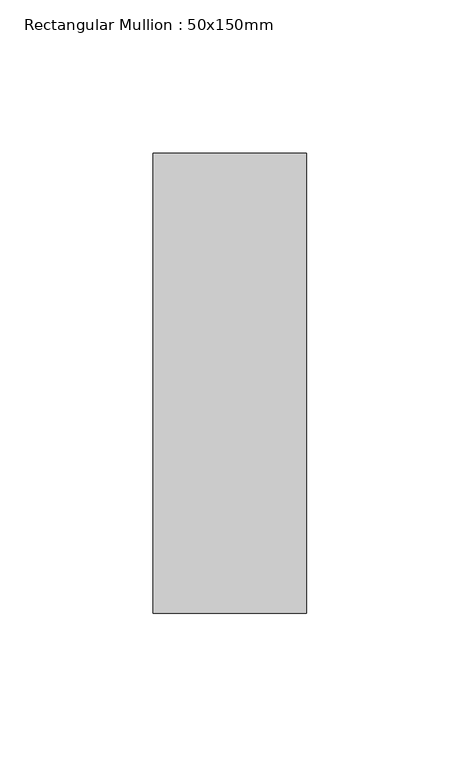
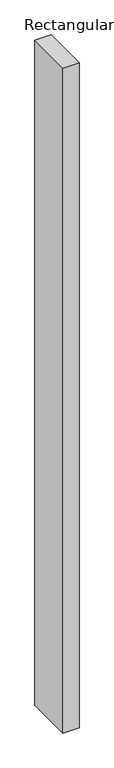
"""IFC4 building model written with IfcOpenShell, lengths in millimetres: member geometry, Rectangular Mullion : 50x150mm."""

from ifc_helpers import new_model, si_unit, frame, origin, place, context, project, spatial, polyline, outline, extrude, source, transform, mapped, element, save


def rectangular_mullion_50x150mm_0a54999a(model_context):
    return source(origin(), model_context, "Body", "SweptSolid", [
        extrude(outline(polyline([(0.0, 75.0), (0.0, -75.0), (-50.0, -75.0), (-50.0, 75.0), (0.0, 75.0)])), frame((0.0, 0.0, -2175.0), z_axis=(0.0, 0.0, 1.0), x_axis=(1.0, 0.0, 0.0)), (0.0, 0.0, 1.0), 2175.0),
    ])


if __name__ == "__main__":
    model = new_model("IFC4")
    model_context = context("Model", 3, world=origin())
    ifc_project = project(units=[si_unit("LENGTHUNIT", "METRE", prefix="MILLI")], contexts=[model_context])
    site = spatial("IfcSite", under=ifc_project)
    building = spatial("IfcBuilding", under=site)
    placement = place(None, origin())
    rectangular_mullion_50x150mm_shape = rectangular_mullion_50x150mm_0a54999a(model_context)
    element("IfcMember", 1, ObjectType="Rectangular Mullion : 50x150mm", at=placement, inside=building, context=model_context, shape_type="MappedRepresentation", body=[
        mapped(rectangular_mullion_50x150mm_shape, transform((0.0, 0.0, 0.0), x_axis=(1.0, 0.0, 0.0), y_axis=(0.0, 1.0, 0.0), z_axis=(0.0, 0.0, 1.0))),
    ])
    save(model, "model.ifc")

# Revit data of these elements
# Type "Rectangular Mullion : 50x150mm"
#   Keynote = "H11"
#   built-in parameter 1007304 = 0.492126 (stored number, unit not read)
#   built-in parameter 1007301 = 0.082021 (stored number, unit not read)
#   built-in parameter 1007300 = 0.082021 (stored number, unit not read)
# Element 1 (IfcMember, "Rectangular Mullion : 50x150mm")
#   Materials on its faces: "Aluminium"
# Materials
#   "Aluminium": class "Metal", colour RGB 247 247 247, transparency 0, Description = "Aluminium 6061", Cost = 0
